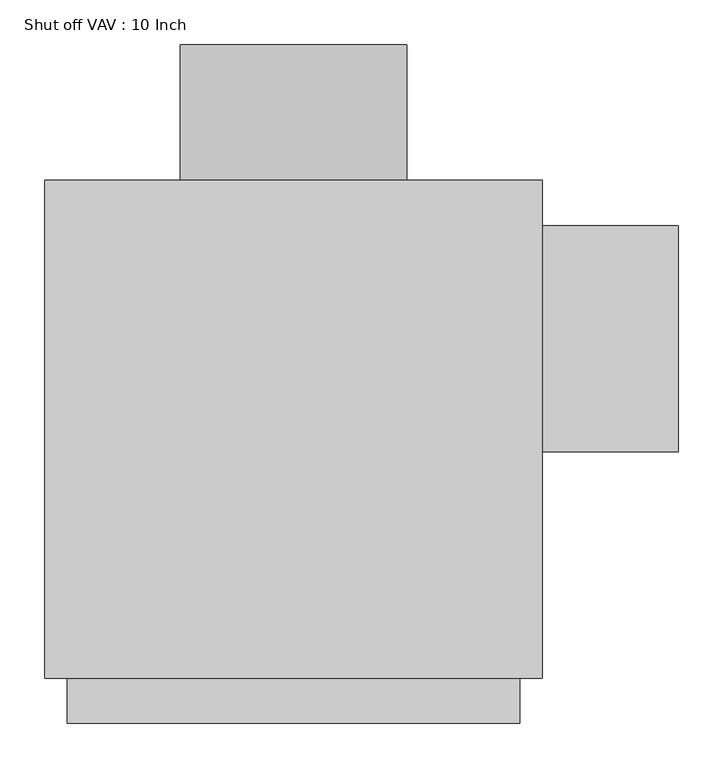
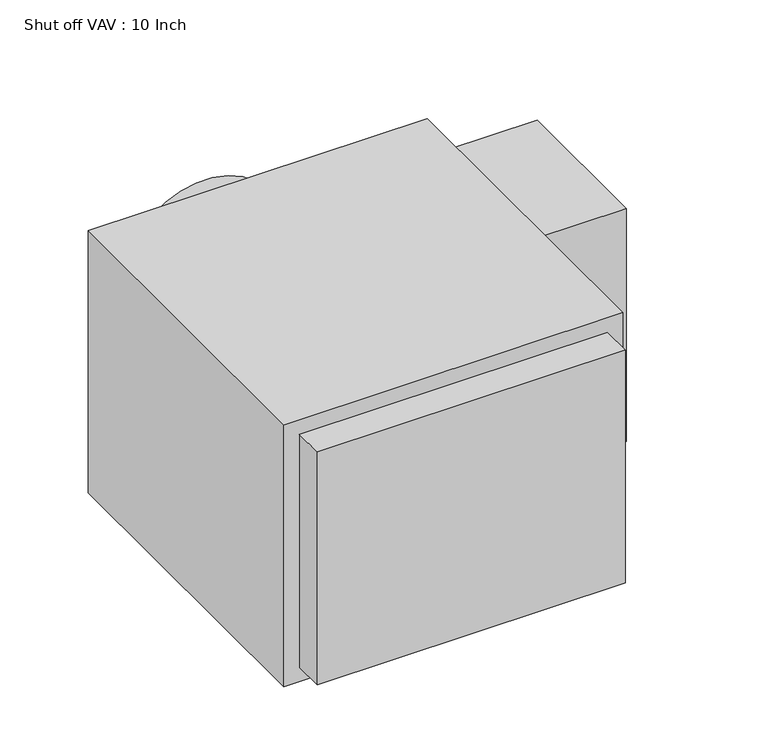
"""IFC4 building model written with IfcOpenShell, lengths in millimetres: proxy geometry, Shut off VAV : 10 Inch."""

from ifc_helpers import new_model, si_unit, point, frame, origin, origin_2d, place, context, project, spatial, polyline, circle_curve, trimmed, segment, composite_curve, outline, extrude, source, transform, mapped, element, save


def shut_off_vav_10_inch_df6e8142(model_context):
    return source(origin(), model_context, "Body", "SweptSolid", [
        extrude(outline(polyline([(431.8, 228.6), (431.8, -25.4), (279.4, -25.4), (279.4, 228.6), (431.8, 228.6)])), frame((0.0, 0.0, -203.2), z_axis=(0.0, 0.0, 1.0), x_axis=(1.0, 0.0, 0.0)), (0.0, 0.0, 1.0), 406.4),
        extrude(outline(composite_curve([segment(trimmed(circle_curve(origin_2d(), 127.0), [point((0.0, -127.0))], [point((0.0, 127.0))], False, "CARTESIAN"), True, "CONTINUOUS"), segment(trimmed(circle_curve(origin_2d(), 127.0), [point((0.0, 127.0))], [point((0.0, -127.0))], False, "CARTESIAN"), True, "CONTINUOUS")], self_intersect=False)), frame((0.0, 279.4, 0.0), z_axis=(0.0, 1.0, 0.0), x_axis=(0.0, 0.0, 1.0)), (0.0, 0.0, 1.0), 152.4),
        extrude(outline(polyline([(254.0, -330.2), (-254.0, -330.2), (-254.0, -279.4), (254.0, -279.4), (254.0, -330.2)])), frame((0.0, 0.0, -203.2), z_axis=(0.0, 0.0, 1.0), x_axis=(1.0, 0.0, 0.0)), (0.0, 0.0, 1.0), 406.4),
        extrude(outline(polyline([(279.4, -279.4), (-279.4, -279.4), (-279.4, 279.4), (279.4, 279.4), (279.4, -279.4)])), frame((0.0, 0.0, -228.6), z_axis=(0.0, 0.0, 1.0), x_axis=(1.0, 0.0, 0.0)), (0.0, 0.0, 1.0), 457.2),
    ])


if __name__ == "__main__":
    model = new_model("IFC4")
    model_context = context("Model", 3, world=origin())
    ifc_project = project(units=[si_unit("LENGTHUNIT", "METRE", prefix="MILLI")], contexts=[model_context])
    site = spatial("IfcSite", under=ifc_project)
    building = spatial("IfcBuilding", under=site)
    placement = place(None, origin())
    shut_off_vav_10_inch_shape = shut_off_vav_10_inch_df6e8142(model_context)
    element("IfcBuildingElementProxy", 1, Name="Shut off VAV : 10 Inch", ObjectType="Shut off VAV : 10 Inch", at=placement, inside=building, context=model_context, shape_type="MappedRepresentation", body=[
        mapped(shut_off_vav_10_inch_shape, transform((0.0, 0.0, 0.0), x_axis=(1.0, 0.0, 0.0), y_axis=(0.0, 1.0, 0.0), z_axis=(0.0, 0.0, 1.0))),
    ])
    save(model, "model.ifc")

# Revit data of these elements
# Type "Shut off VAV : 10 Inch"
#   UnitWidth = 1' - 10"
#   UnitLength = 1' - 10"
#   UnitHeight = 1' - 6"
#   SupplyWidth = 1' - 8"
#   SupplyHeight = 1' - 4"
#   Static Pressure Drop [instance default] = 0.00 in-wg
#   PrimaryRadius = 0' - 5"
#   PrimaryLength = 1' - 5"
#   OuterControlWidth = 1' - 5"
#   HalfUnitHeight = 0' - 9"
#   HalfSupplyHeight = 0' - 8"
#   Air Flow [instance default] = 0 CFM
#   Assembly Code = ""
# Element 1 (IfcBuildingElementProxy, "Shut off VAV : 10 Inch")
#   Static Pressure Drop = 0.09 in-wg
#   Air Flow = 1180 CFM
